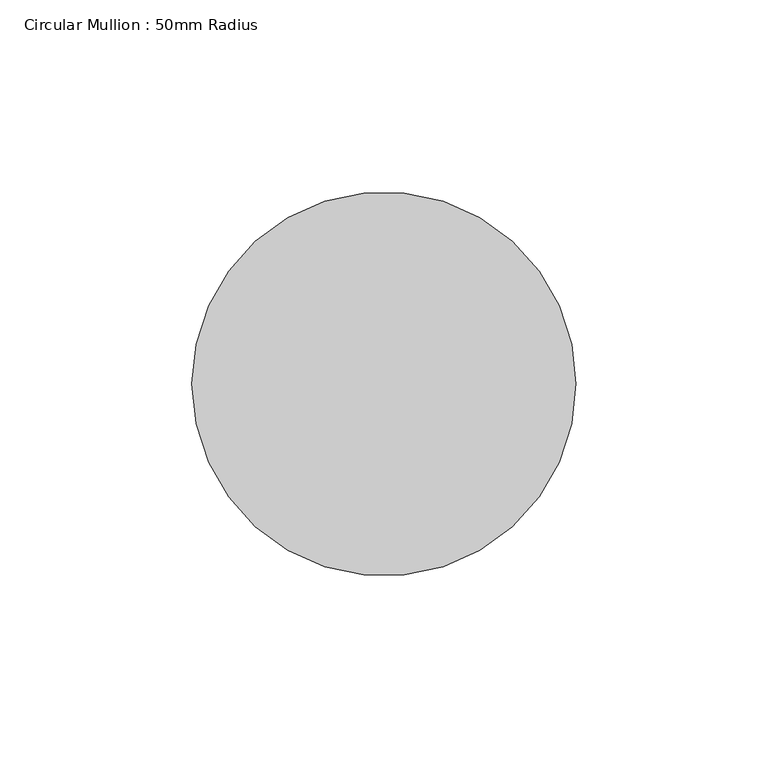
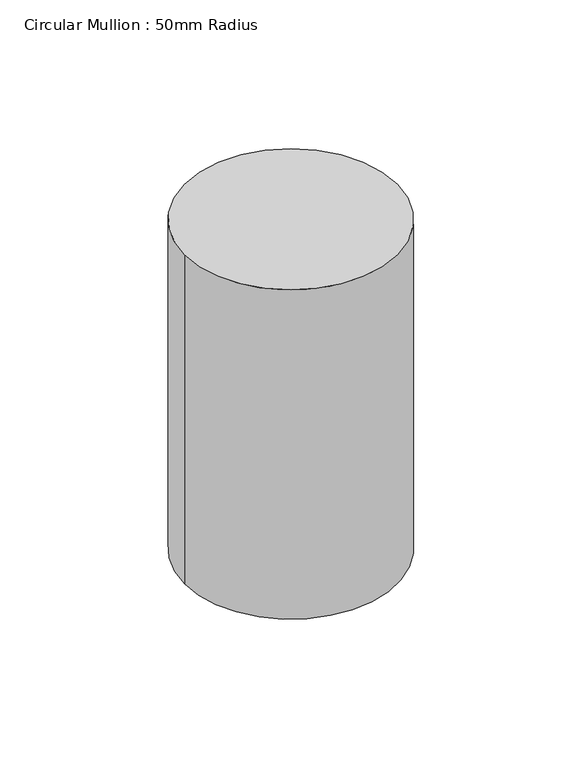
"""IFC4 building model written with IfcOpenShell, lengths in millimetres: member geometry, Circular Mullion : 50mm Radius."""

from ifc_helpers import new_model, si_unit, point, frame, origin, origin_2d, place, context, project, spatial, circle_curve, trimmed, segment, composite_curve, outline, extrude, source, transform, mapped, element, save


def circular_mullion_50mm_radius_9ead6e7c(model_context):
    return source(origin(), model_context, "Body", "SweptSolid", [
        extrude(outline(composite_curve([segment(trimmed(circle_curve(origin_2d(), 50.0), [point((50.0, 0.0))], [point((-50.0, 0.0))], False, "CARTESIAN"), True, "CONTINUOUS"), segment(trimmed(circle_curve(origin_2d(), 50.0), [point((-50.0, 0.0))], [point((50.0, 0.0))], False, "CARTESIAN"), True, "CONTINUOUS")], self_intersect=False)), frame((0.0, 0.0, -163.3568527), z_axis=(0.0, 0.0, 1.0), x_axis=(1.0, 0.0, 0.0)), (0.0, 0.0, 1.0), 163.3568527),
    ])


if __name__ == "__main__":
    model = new_model("IFC4")
    model_context = context("Model", 3, world=origin())
    ifc_project = project(units=[si_unit("LENGTHUNIT", "METRE", prefix="MILLI")], contexts=[model_context])
    site = spatial("IfcSite", under=ifc_project)
    building = spatial("IfcBuilding", under=site)
    placement = place(None, origin())
    circular_mullion_50mm_radius_shape = circular_mullion_50mm_radius_9ead6e7c(model_context)
    element("IfcMember", 1, ObjectType="Circular Mullion : 50mm Radius", at=placement, inside=building, context=model_context, shape_type="MappedRepresentation", body=[
        mapped(circular_mullion_50mm_radius_shape, transform((0.0, 0.0, 0.0), x_axis=(1.0, 0.0, 0.0), y_axis=(0.0, 1.0, 0.0), z_axis=(0.0, 0.0, 1.0))),
    ])
    save(model, "model.ifc")

# Revit data of these elements
# Type "Circular Mullion : 50mm Radius"
#   built-in parameter 1007350 = 0.164042 (stored number, unit not read)
# Element 1 (IfcMember, "Circular Mullion : 50mm Radius")
#   Materials on its faces: "Aluminium"
# Materials
#   "Aluminium": class "Metal", colour RGB 247 247 247, transparency 0, Description = "Aluminium 6061", Cost = 0
